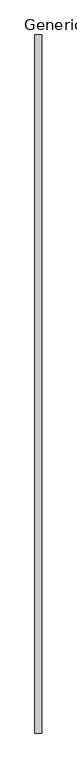
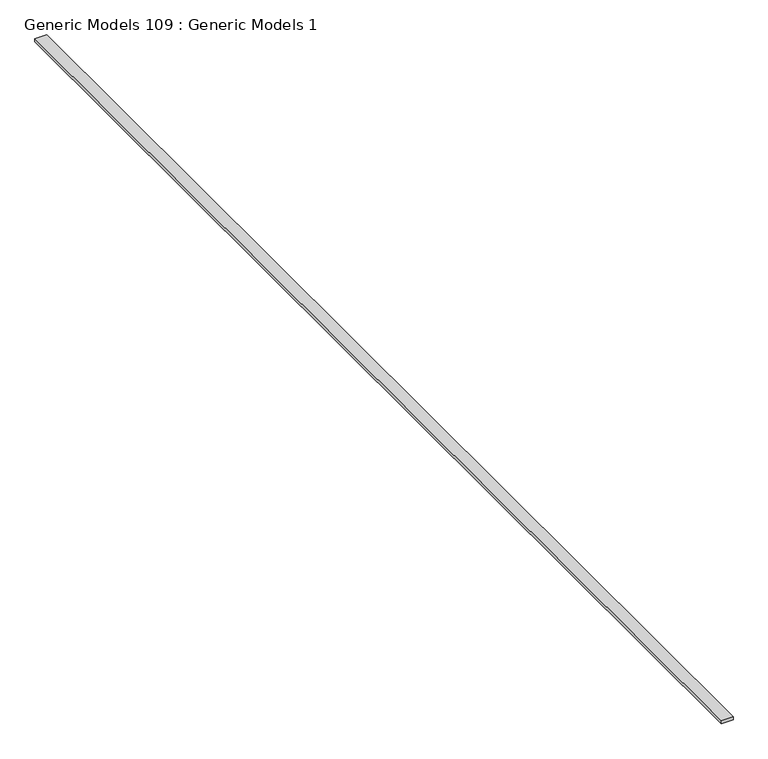
"""IFC4 building model written with IfcOpenShell, lengths in millimetres: proxy geometry, Generic Models 109 : Generic Models 1."""

from ifc_helpers import new_model, si_unit, frame, origin, place, context, project, spatial, polyline, outline, extrude, source, transform, mapped, element, save


def generic_models_109_generic_models_1_a83170d0(model_context):
    return source(origin(), model_context, "Body", "SweptSolid", [
        extrude(outline(polyline([(-6005.2146508, 7054.2769662), (-5865.5146508, 7054.2769662), (-5865.5146508, -7068.1230338), (-6005.2146508, -7068.1230338), (-6005.2146508, 7054.2769662)])), frame((0.0, 0.0, 126039.3883865), z_axis=(0.0, 0.0, 1.0), x_axis=(1.0, 0.0, 0.0)), (0.0, 0.0, 1.0), 38.1),
    ])


if __name__ == "__main__":
    model = new_model("IFC4")
    model_context = context("Model", 3, world=origin())
    ifc_project = project(units=[si_unit("LENGTHUNIT", "METRE", prefix="MILLI")], contexts=[model_context])
    site = spatial("IfcSite", under=ifc_project)
    building = spatial("IfcBuilding", under=site)
    placement = place(None, origin())
    generic_models_109_generic_models_1_shape = generic_models_109_generic_models_1_a83170d0(model_context)
    element("IfcBuildingElementProxy", 1, Name="Generic Models 109 : Generic Models 1", ObjectType="Generic Models 109 : Generic Models 1", at=placement, inside=building, context=model_context, shape_type="MappedRepresentation", body=[
        mapped(generic_models_109_generic_models_1_shape, transform((0.0, 0.0, 0.0), x_axis=(1.0, 0.0, 0.0), y_axis=(0.0, 1.0, 0.0), z_axis=(0.0, 0.0, 1.0))),
    ])
    save(model, "model.ifc")

# Revit data of these elements
# Element 1 (IfcBuildingElementProxy, "Generic Models 109 : Generic Models 1")
#   Materials on its faces: "_2X BLOCKING AS REQUIRED"
# Materials
#   "_2X BLOCKING AS REQUIRED": class "Generic", colour RGB 177 130 114, transparency 0, Cost = 0
